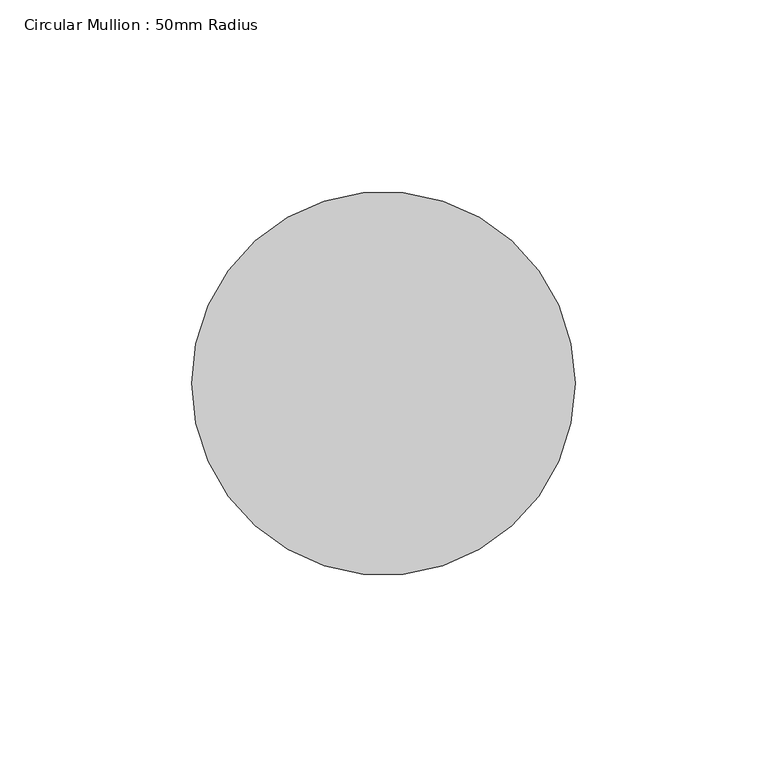
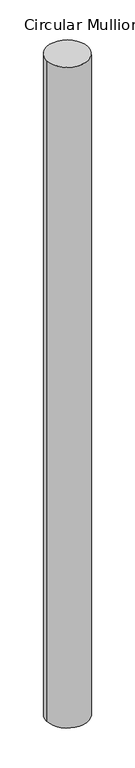
"""IFC4 building model written with IfcOpenShell, lengths in millimetres: member geometry, Circular Mullion : 50mm Radius."""

from ifc_helpers import new_model, si_unit, point, frame, origin, origin_2d, place, context, project, spatial, circle_curve, trimmed, segment, composite_curve, outline, extrude, source, transform, mapped, element, save


def circular_mullion_50mm_radius_6f2b6d1d(model_context):
    return source(origin(), model_context, "Body", "SweptSolid", [
        extrude(outline(composite_curve([segment(trimmed(circle_curve(origin_2d(), 50.0), [point((50.0, 0.0))], [point((-50.0, 0.0))], False, "CARTESIAN"), True, "CONTINUOUS"), segment(trimmed(circle_curve(origin_2d(), 50.0), [point((-50.0, 0.0))], [point((50.0, 0.0))], False, "CARTESIAN"), True, "CONTINUOUS")], self_intersect=False)), frame((0.0, 0.0, -1684.074463), z_axis=(0.0, 0.0, 1.0), x_axis=(1.0, 0.0, 0.0)), (0.0, 0.0, 1.0), 1684.074463),
    ])


if __name__ == "__main__":
    model = new_model("IFC4")
    model_context = context("Model", 3, world=origin())
    ifc_project = project(units=[si_unit("LENGTHUNIT", "METRE", prefix="MILLI")], contexts=[model_context])
    site = spatial("IfcSite", under=ifc_project)
    building = spatial("IfcBuilding", under=site)
    placement = place(None, origin())
    circular_mullion_50mm_radius_shape = circular_mullion_50mm_radius_6f2b6d1d(model_context)
    element("IfcMember", 1, ObjectType="Circular Mullion : 50mm Radius", at=placement, inside=building, context=model_context, shape_type="MappedRepresentation", body=[
        mapped(circular_mullion_50mm_radius_shape, transform((0.0, 0.0, 0.0), x_axis=(1.0, 0.0, 0.0), y_axis=(0.0, 1.0, 0.0), z_axis=(0.0, 0.0, 1.0))),
    ])
    save(model, "model.ifc")

# Revit data of these elements
# Type "Circular Mullion : 50mm Radius"
#   built-in parameter 1007350 = 0.164042 (stored number, unit not read)
# Element 1 (IfcMember, "Circular Mullion : 50mm Radius")
#   Materials on its faces: "Aluminium"
# Materials
#   "Aluminium": class "Metal", colour RGB 247 247 247, transparency 0, Description = "Aluminium 6061", Cost = 0
